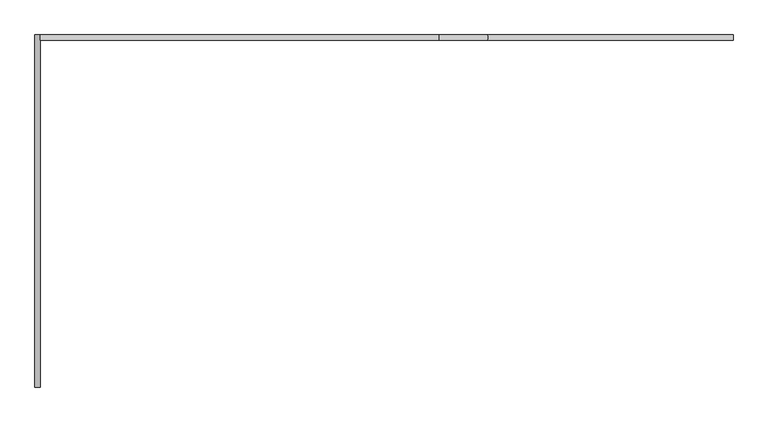
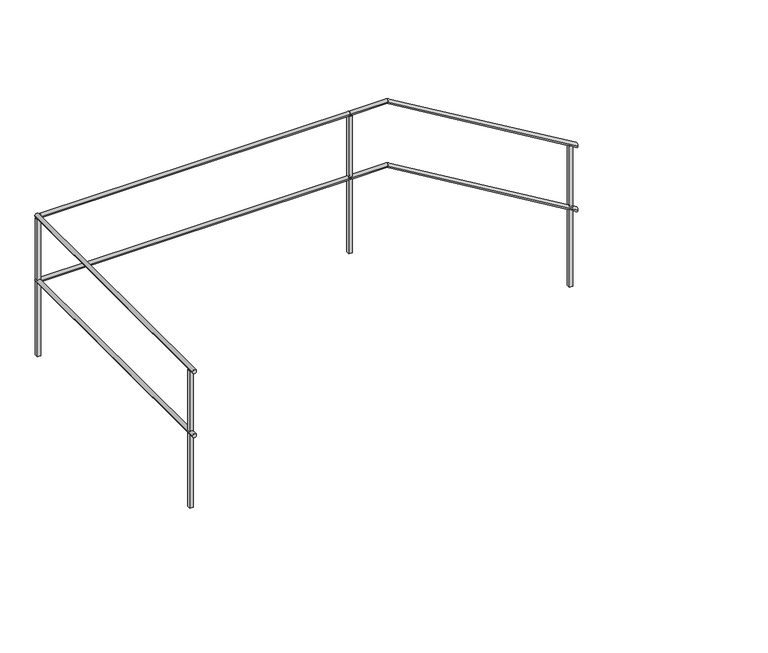
"""IFC4 building model written with IfcOpenShell, lengths in millimetres: railing geometry."""

from ifc_helpers import new_model, si_unit, frame, origin, place, context, project, spatial, polyline, circle_curve, ellipse_curve, outline, extrude, source, transform, mapped, element, save
from ifc_brep_helpers import plane_surface, cylinder_surface, advanced_brep


def railing_8ab6cbfe(model_context):
    return source(origin(), model_context, "Body", "SolidModel", [
        advanced_brep(
        [(33043.8956602, 25734.1208589, 899.1723166), (33043.8956602, 25764.1208589, 899.1723166), (31639.7692216, 25734.1208589, 1734.9618634), (31639.7692216, 25764.1208589, 1734.9618634), (31363.8956602, 25734.1208589, 1734.9618634), (31363.8956602, 25764.1208589, 1734.9618634)],
        [
            (0, 1, ellipse_curve(frame((33043.8956602, 25749.1208589, 899.1723166), z_axis=(1.0, 0.0, 0.0), x_axis=(0.0, 0.0, -1.0)), 17.4562134, 15.0)),
            (1, 0, ellipse_curve(frame((33043.8956602, 25749.1208589, 899.1723166), z_axis=(1.0, 0.0, 0.0), x_axis=(0.0, 0.0, -1.0)), 17.4562134, 15.0)),
            (0, 2),
            (2, 3, ellipse_curve(frame((31639.7692216, 25749.1208589, 1734.9618634), z_axis=(0.9641817474962142, 0.0, -0.26524245096731175), x_axis=(-0.26524245096731197, 0.0, -0.964181747496214)), 15.5572329, 15.0)),
            (3, 1),
            (3, 2, ellipse_curve(frame((31639.7692216, 25749.1208589, 1734.9618634), z_axis=(0.9641817474962142, 0.0, -0.26524245096731175), x_axis=(-0.26524245096731197, 0.0, -0.964181747496214)), 15.5572329, 15.0)),
            (4, 5, circle_curve(frame((31363.8956602, 25749.1208589, 1734.9618634), z_axis=(-1.0, 0.0, 0.0), x_axis=(0.0, 1.0, 0.0)), 15.0)),
            (5, 4, circle_curve(frame((31363.8956602, 25749.1208589, 1734.9618634), z_axis=(-1.0, 0.0, 0.0), x_axis=(0.0, 1.0, 0.0)), 15.0)),
            (2, 4),
            (5, 3),
        ],
        [
            plane_surface(frame((33043.8956602, 25749.1208589, 916.62853), z_axis=(1.0, 0.0, 0.0), x_axis=(0.0, -1.0, 0.0))),
            cylinder_surface(frame((33036.2234023, 25749.1208589, 903.7391368), z_axis=(0.8592928844097065, 0.0, -0.5114838597676831), x_axis=(0.0, 1.0, 0.0)), 15.0),
            plane_surface(frame((31363.8956602, 25749.1208589, 1749.9618634), z_axis=(-1.0, 0.0, 0.0), x_axis=(0.0, -1.0, 0.0))),
            cylinder_surface(frame((31643.8956602, 25749.1208589, 1734.9618634), z_axis=(1.0, 0.0, 0.0), x_axis=(0.0, 1.0, 0.0)), 15.0),
        ],
        [
            (0, [[1, 2]]),
            (1, [[-1, 3, 4, 5]]),
            (1, [[-2, -5, 6, -3]]),
            (2, [[7, 8]]),
            (3, [[-4, 9, -8, 10]]),
            (3, [[-6, -10, -7, -9]]),
        ],
    ),
        advanced_brep(
        [(31363.8956602, 25734.1208589, 1734.9618634), (31363.8956602, 25764.1208589, 1734.9618634), (29079.2956602, 25734.1208589, 1734.9618634), (29079.2956602, 25764.1208589, 1734.9618634)],
        [
            (0, 1, circle_curve(frame((31363.8956602, 25749.1208589, 1734.9618634), z_axis=(1.0, 0.0, 0.0), x_axis=(0.0, 1.0, 0.0)), 15.0)),
            (1, 0, circle_curve(frame((31363.8956602, 25749.1208589, 1734.9618634), z_axis=(1.0, 0.0, 0.0), x_axis=(0.0, 1.0, 0.0)), 15.0)),
            (2, 3, circle_curve(frame((29079.2956602, 25749.1208589, 1734.9618634), z_axis=(-1.0, 0.0, 0.0), x_axis=(0.0, 1.0, 0.0)), 15.0)),
            (3, 2, circle_curve(frame((29079.2956602, 25749.1208589, 1734.9618634), z_axis=(-1.0, 0.0, 0.0), x_axis=(0.0, 1.0, 0.0)), 15.0)),
            (0, 2),
            (3, 1),
        ],
        [
            plane_surface(frame((31363.8956602, 25749.1208589, 1749.9618634), z_axis=(1.0, 0.0, 0.0), x_axis=(0.0, -1.0, 0.0))),
            plane_surface(frame((29079.2956602, 25749.1208589, 1749.9618634), z_axis=(-1.0, 0.0, 0.0), x_axis=(0.0, -1.0, 0.0))),
            cylinder_surface(frame((31363.8956602, 25749.1208589, 1734.9618634), z_axis=(1.0, 0.0, 0.0), x_axis=(0.0, 1.0, 0.0)), 15.0),
        ],
        [
            (0, [[1, 2]]),
            (1, [[3, 4]]),
            (2, [[-1, 5, -4, 6]]),
            (2, [[-2, -6, -3, -5]]),
        ],
    ),
        advanced_brep(
        [(29079.2956602, 25764.1208589, 1734.9618634), (29049.2956602, 25764.1208589, 1734.9618634), (29079.2956602, 23749.5208589, 1734.9618634), (29049.2956602, 23749.5208589, 1734.9618634)],
        [
            (0, 1, circle_curve(frame((29064.2956602, 25764.1208589, 1734.9618634), z_axis=(0.0, 1.0, 0.0), x_axis=(-1.0, 0.0, 0.0)), 15.0)),
            (1, 0, circle_curve(frame((29064.2956602, 25764.1208589, 1734.9618634), z_axis=(0.0, 1.0, 0.0), x_axis=(-1.0, 0.0, 0.0)), 15.0)),
            (2, 3, circle_curve(frame((29064.2956602, 23749.5208589, 1734.9618634), z_axis=(0.0, -1.0, 0.0), x_axis=(-1.0, 0.0, 0.0)), 15.0)),
            (3, 2, circle_curve(frame((29064.2956602, 23749.5208589, 1734.9618634), z_axis=(0.0, -1.0, 0.0), x_axis=(-1.0, 0.0, 0.0)), 15.0)),
            (0, 2),
            (3, 1),
        ],
        [
            plane_surface(frame((29064.2956602, 25764.1208589, 1749.9618634), z_axis=(0.0, 1.0, 0.0), x_axis=(0.0, 0.0, -1.0))),
            plane_surface(frame((29064.2956602, 23749.5208589, 1749.9618634), z_axis=(0.0, -1.0, 0.0), x_axis=(0.0, 0.0, -1.0))),
            cylinder_surface(frame((29064.2956602, 25764.1208589, 1734.9618634), z_axis=(0.0, 1.0, 0.0), x_axis=(-1.0, 0.0, 0.0)), 15.0),
        ],
        [
            (0, [[1, 2]]),
            (1, [[3, 4]]),
            (2, [[-1, 5, -4, 6]]),
            (2, [[-2, -6, -3, -5]]),
        ],
    ),
        advanced_brep(
        [(33043.8956602, 25734.1208589, 1399.1723166), (33043.8956602, 25764.1208589, 1399.1723166), (31639.7692216, 25734.1208589, 2234.9618634), (31639.7692216, 25764.1208589, 2234.9618634), (31363.8956602, 25734.1208589, 2234.9618634), (31363.8956602, 25764.1208589, 2234.9618634)],
        [
            (0, 1, ellipse_curve(frame((33043.8956602, 25749.1208589, 1399.1723166), z_axis=(1.0, 0.0, 0.0), x_axis=(0.0, 0.0, -1.0)), 17.4562134, 15.0)),
            (1, 0, ellipse_curve(frame((33043.8956602, 25749.1208589, 1399.1723166), z_axis=(1.0, 0.0, 0.0), x_axis=(0.0, 0.0, -1.0)), 17.4562134, 15.0)),
            (0, 2),
            (2, 3, ellipse_curve(frame((31639.7692216, 25749.1208589, 2234.9618634), z_axis=(0.9641817474962142, 0.0, -0.26524245096731175), x_axis=(-0.26524245096731197, 0.0, -0.964181747496214)), 15.5572329, 15.0)),
            (3, 1),
            (3, 2, ellipse_curve(frame((31639.7692216, 25749.1208589, 2234.9618634), z_axis=(0.9641817474962142, 0.0, -0.26524245096731175), x_axis=(-0.26524245096731197, 0.0, -0.964181747496214)), 15.5572329, 15.0)),
            (4, 5, circle_curve(frame((31363.8956602, 25749.1208589, 2234.9618634), z_axis=(-1.0, 0.0, 0.0), x_axis=(0.0, 1.0, 0.0)), 15.0)),
            (5, 4, circle_curve(frame((31363.8956602, 25749.1208589, 2234.9618634), z_axis=(-1.0, 0.0, 0.0), x_axis=(0.0, 1.0, 0.0)), 15.0)),
            (2, 4),
            (5, 3),
        ],
        [
            plane_surface(frame((33043.8956602, 25749.1208589, 1416.62853), z_axis=(1.0, 0.0, 0.0), x_axis=(0.0, -1.0, 0.0))),
            cylinder_surface(frame((33036.2234023, 25749.1208589, 1403.7391368), z_axis=(0.8592928844097065, 0.0, -0.5114838597676831), x_axis=(0.0, 1.0, 0.0)), 15.0),
            plane_surface(frame((31363.8956602, 25749.1208589, 2249.9618634), z_axis=(-1.0, 0.0, 0.0), x_axis=(0.0, -1.0, 0.0))),
            cylinder_surface(frame((31643.8956602, 25749.1208589, 2234.9618634), z_axis=(1.0, 0.0, 0.0), x_axis=(0.0, 1.0, 0.0)), 15.0),
        ],
        [
            (0, [[1, 2]]),
            (1, [[-1, 3, 4, 5]]),
            (1, [[-2, -5, 6, -3]]),
            (2, [[7, 8]]),
            (3, [[-4, 9, -8, 10]]),
            (3, [[-6, -10, -7, -9]]),
        ],
    ),
        advanced_brep(
        [(31363.8956602, 25734.1208589, 2234.9618634), (31363.8956602, 25764.1208589, 2234.9618634), (29079.2956602, 25734.1208589, 2234.9618634), (29079.2956602, 25764.1208589, 2234.9618634)],
        [
            (0, 1, circle_curve(frame((31363.8956602, 25749.1208589, 2234.9618634), z_axis=(1.0, 0.0, 0.0), x_axis=(0.0, 1.0, 0.0)), 15.0)),
            (1, 0, circle_curve(frame((31363.8956602, 25749.1208589, 2234.9618634), z_axis=(1.0, 0.0, 0.0), x_axis=(0.0, 1.0, 0.0)), 15.0)),
            (2, 3, circle_curve(frame((29079.2956602, 25749.1208589, 2234.9618634), z_axis=(-1.0, 0.0, 0.0), x_axis=(0.0, 1.0, 0.0)), 15.0)),
            (3, 2, circle_curve(frame((29079.2956602, 25749.1208589, 2234.9618634), z_axis=(-1.0, 0.0, 0.0), x_axis=(0.0, 1.0, 0.0)), 15.0)),
            (0, 2),
            (3, 1),
        ],
        [
            plane_surface(frame((31363.8956602, 25749.1208589, 2249.9618634), z_axis=(1.0, 0.0, 0.0), x_axis=(0.0, -1.0, 0.0))),
            plane_surface(frame((29079.2956602, 25749.1208589, 2249.9618634), z_axis=(-1.0, 0.0, 0.0), x_axis=(0.0, -1.0, 0.0))),
            cylinder_surface(frame((31363.8956602, 25749.1208589, 2234.9618634), z_axis=(1.0, 0.0, 0.0), x_axis=(0.0, 1.0, 0.0)), 15.0),
        ],
        [
            (0, [[1, 2]]),
            (1, [[3, 4]]),
            (2, [[-1, 5, -4, 6]]),
            (2, [[-2, -6, -3, -5]]),
        ],
    ),
        advanced_brep(
        [(29079.2956602, 25764.1208589, 2234.9618634), (29049.2956602, 25764.1208589, 2234.9618634), (29079.2956602, 23749.5208589, 2234.9618634), (29049.2956602, 23749.5208589, 2234.9618634)],
        [
            (0, 1, circle_curve(frame((29064.2956602, 25764.1208589, 2234.9618634), z_axis=(0.0, 1.0, 0.0), x_axis=(-1.0, 0.0, 0.0)), 15.0)),
            (1, 0, circle_curve(frame((29064.2956602, 25764.1208589, 2234.9618634), z_axis=(0.0, 1.0, 0.0), x_axis=(-1.0, 0.0, 0.0)), 15.0)),
            (2, 3, circle_curve(frame((29064.2956602, 23749.5208589, 2234.9618634), z_axis=(0.0, -1.0, 0.0), x_axis=(-1.0, 0.0, 0.0)), 15.0)),
            (3, 2, circle_curve(frame((29064.2956602, 23749.5208589, 2234.9618634), z_axis=(0.0, -1.0, 0.0), x_axis=(-1.0, 0.0, 0.0)), 15.0)),
            (0, 2),
            (3, 1),
        ],
        [
            plane_surface(frame((29064.2956602, 25764.1208589, 2249.9618634), z_axis=(0.0, 1.0, 0.0), x_axis=(0.0, 0.0, -1.0))),
            plane_surface(frame((29064.2956602, 23749.5208589, 2249.9618634), z_axis=(0.0, -1.0, 0.0), x_axis=(0.0, 0.0, -1.0))),
            cylinder_surface(frame((29064.2956602, 25764.1208589, 2234.9618634), z_axis=(0.0, 1.0, 0.0), x_axis=(-1.0, 0.0, 0.0)), 15.0),
        ],
        [
            (0, [[1, 2]]),
            (1, [[3, 4]]),
            (2, [[-1, 5, -4, 6]]),
            (2, [[-2, -6, -3, -5]]),
        ],
    ),
        extrude(outline(polyline([(29076.7956602, 25761.6208589), (29076.7956602, 25736.6208589), (29051.7956602, 25736.6208589), (29051.7956602, 25761.6208589), (29076.7956602, 25761.6208589)])), frame((0.0, 0.0, 1149.9618634), z_axis=(0.0, 0.0, 1.0), x_axis=(1.0, 0.0, 0.0)), (0.0, 0.0, 1.0), 1070.0),
        extrude(outline(polyline([(31376.3956602, 25761.6208589), (31376.3956602, 25736.6208589), (31351.3956602, 25736.6208589), (31351.3956602, 25761.6208589), (31376.3956602, 25761.6208589)])), frame((0.0, 0.0, 1149.9618634), z_axis=(0.0, 0.0, 1.0), x_axis=(1.0, 0.0, 0.0)), (0.0, 0.0, 1.0), 1070.0),
        extrude(outline(polyline([(29051.7956602, 23812.0208589), (29076.7956602, 23812.0208589), (29076.7956602, 23787.0208589), (29051.7956602, 23787.0208589), (29051.7956602, 23812.0208589)])), frame((0.0, 0.0, 1149.9618634), z_axis=(0.0, 0.0, 1.0), x_axis=(1.0, 0.0, 0.0)), (0.0, 0.0, 1.0), 1070.0),
        extrude(outline(polyline([(316.62853, 33006.3956602), (1408.9499586, 33006.3956602), (1423.830911, 32981.3956602), (316.62853, 32981.3956602), (316.62853, 33006.3956602)])), frame((0.0, 25736.6208589, 0.0), z_axis=(0.0, 1.0, 0.0), x_axis=(0.0, 0.0, 1.0)), (0.0, 0.0, 1.0), 25.0),
    ])


if __name__ == "__main__":
    model = new_model("IFC4")
    model_context = context("Model", 3, world=origin())
    ifc_project = project(units=[si_unit("LENGTHUNIT", "METRE", prefix="MILLI")], contexts=[model_context])
    site = spatial("IfcSite", under=ifc_project)
    building = spatial("IfcBuilding", under=site)
    placement = place(None, origin())
    railing_shape = railing_8ab6cbfe(model_context)
    element("IfcRailing", 1, at=placement, inside=building, context=model_context, shape_type="MappedRepresentation", body=[
        mapped(railing_shape, transform((0.0, 0.0, 0.0), x_axis=(1.0, 0.0, 0.0), y_axis=(0.0, 1.0, 0.0), z_axis=(0.0, 0.0, 1.0))),
    ])
    save(model, "model.ifc")
